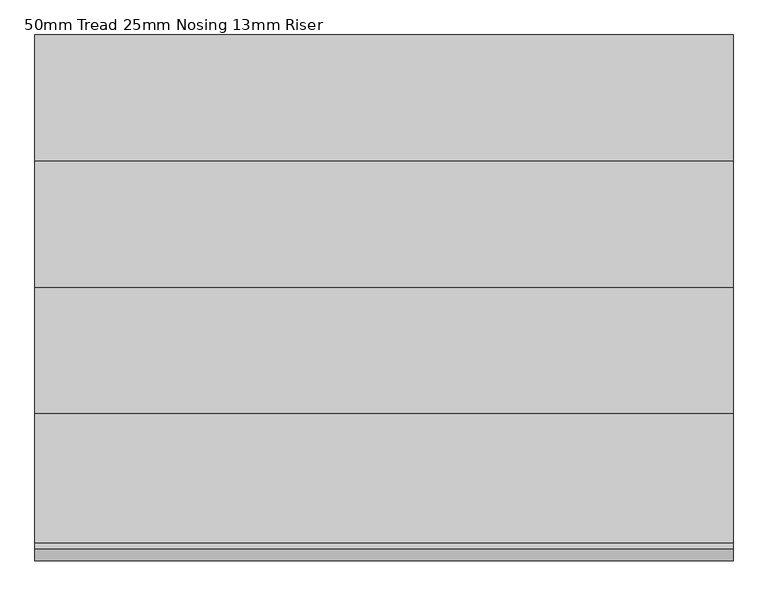
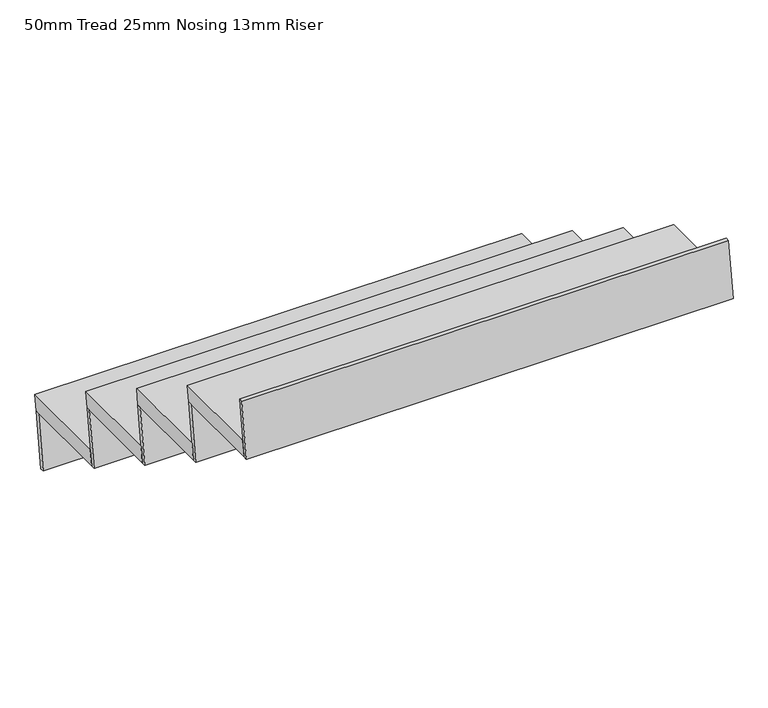
"""IFC4 building model written with IfcOpenShell, lengths in millimetres: stair flight geometry, 50mm Tread 25mm Nosing 13mm Riser."""

from ifc_helpers import new_model, si_unit, frame, origin, place, context, project, spatial, polyline, outline, extrude, source, transform, mapped, element, save


def stair_flight_50mm_tread_25mm_nosing_13mm_riser_25054bb9(model_context):
    return source(origin(), model_context, "Body", "SweptSolid", [
        extrude(outline(polyline([(7032.4781803, 17794.1176471), (7332.4781803, 17794.1176471), (7325.3948469, 17744.1176471), (7025.3948469, 17744.1176471), (7032.4781803, 17794.1176471)])), frame((-226.7120949, 0.0, 0.0), z_axis=(1.0, 0.0, 0.0), x_axis=(0.0, 1.0, 0.0)), (0.0, 0.0, 1.0), 1520.0),
        extrude(outline(polyline([(7325.3948469, 17744.1176471), (7300.3948469, 17567.6470588), (7287.770036, 17567.6470588), (7312.770036, 17744.1176471), (7325.3948469, 17744.1176471)])), frame((-226.7120949, 0.0, 0.0), z_axis=(1.0, 0.0, 0.0), x_axis=(0.0, 1.0, 0.0)), (0.0, 0.0, 1.0), 1520.0),
        extrude(outline(polyline([(7050.3948469, 17920.5882353), (7025.3948469, 17744.1176471), (7012.770036, 17744.1176471), (7037.770036, 17920.5882353), (7050.3948469, 17920.5882353)])), frame((-226.7120949, 0.0, 0.0), z_axis=(1.0, 0.0, 0.0), x_axis=(0.0, 1.0, 0.0)), (0.0, 0.0, 1.0), 1520.0),
        extrude(outline(polyline([(6757.4781803, 17970.5882353), (7057.4781803, 17970.5882353), (7050.3948469, 17920.5882353), (6750.3948469, 17920.5882353), (6757.4781803, 17970.5882353)])), frame((-226.7120949, 0.0, 0.0), z_axis=(1.0, 0.0, 0.0), x_axis=(0.0, 1.0, 0.0)), (0.0, 0.0, 1.0), 1520.0),
        extrude(outline(polyline([(6775.3948469, 18097.0588235), (6750.3948469, 17920.5882353), (6737.770036, 17920.5882353), (6762.770036, 18097.0588235), (6775.3948469, 18097.0588235)])), frame((-226.7120949, 0.0, 0.0), z_axis=(1.0, 0.0, 0.0), x_axis=(0.0, 1.0, 0.0)), (0.0, 0.0, 1.0), 1520.0),
        extrude(outline(polyline([(6482.4781803, 18147.0588235), (6782.4781803, 18147.0588235), (6775.3948469, 18097.0588235), (6475.3948469, 18097.0588235), (6482.4781803, 18147.0588235)])), frame((-226.7120949, 0.0, 0.0), z_axis=(1.0, 0.0, 0.0), x_axis=(0.0, 1.0, 0.0)), (0.0, 0.0, 1.0), 1520.0),
        extrude(outline(polyline([(6500.3948469, 18273.5294118), (6475.3948469, 18097.0588235), (6462.770036, 18097.0588235), (6487.770036, 18273.5294118), (6500.3948469, 18273.5294118)])), frame((-226.7120949, 0.0, 0.0), z_axis=(1.0, 0.0, 0.0), x_axis=(0.0, 1.0, 0.0)), (0.0, 0.0, 1.0), 1520.0),
        extrude(outline(polyline([(6225.3948469, 18450.0), (6200.3948469, 18273.5294118), (6187.770036, 18273.5294118), (6212.770036, 18450.0), (6225.3948469, 18450.0)])), frame((-226.7120949, 0.0, 0.0), z_axis=(1.0, 0.0, 0.0), x_axis=(0.0, 1.0, 0.0)), (0.0, 0.0, 1.0), 1520.0),
        extrude(outline(polyline([(6207.4781803, 18323.5294118), (6507.4781803, 18323.5294118), (6500.3948469, 18273.5294118), (6200.3948469, 18273.5294118), (6207.4781803, 18323.5294118)])), frame((-226.7120949, 0.0, 0.0), z_axis=(1.0, 0.0, 0.0), x_axis=(0.0, 1.0, 0.0)), (0.0, 0.0, 1.0), 1520.0),
    ])


if __name__ == "__main__":
    model = new_model("IFC4")
    model_context = context("Model", 3, world=origin())
    ifc_project = project(units=[si_unit("LENGTHUNIT", "METRE", prefix="MILLI")], contexts=[model_context])
    site = spatial("IfcSite", under=ifc_project)
    building = spatial("IfcBuilding", under=site)
    placement = place(None, origin())
    stair_flight_50mm_tread_25mm_nosing_13mm_riser_shape = stair_flight_50mm_tread_25mm_nosing_13mm_riser_25054bb9(model_context)
    element("IfcStairFlight", 1, ObjectType="50mm Tread 25mm Nosing 13mm Riser", at=placement, inside=building, context=model_context, shape_type="MappedRepresentation", body=[
        mapped(stair_flight_50mm_tread_25mm_nosing_13mm_riser_shape, transform((0.0, 0.0, 0.0), x_axis=(1.0, 0.0, 0.0), y_axis=(0.0, 1.0, 0.0), z_axis=(0.0, 0.0, 1.0))),
    ])
    save(model, "model.ifc")
